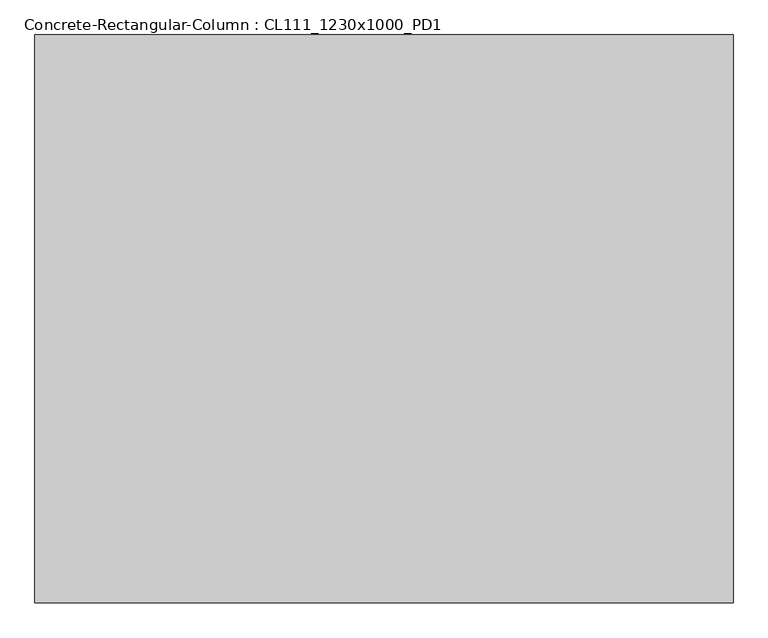
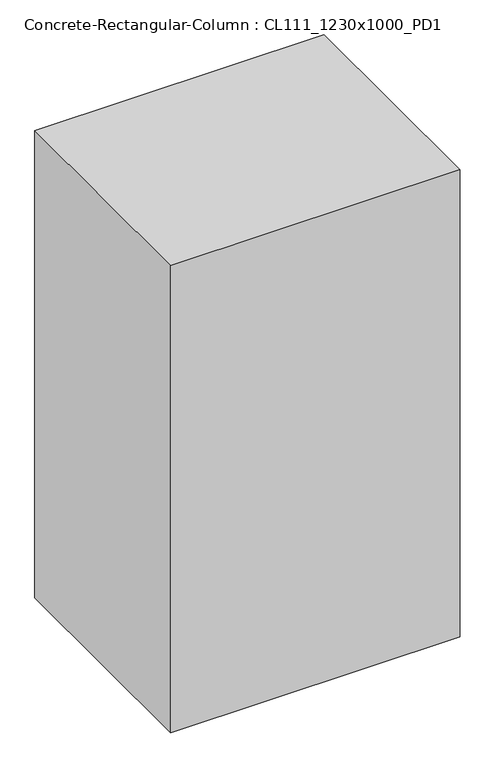
"""IFC4 building model written with IfcOpenShell, lengths in millimetres: column geometry, Concrete-Rectangular-Column : CL111_1230x1000_PD1."""

from ifc_helpers import new_model, si_unit, frame, origin, place, context, project, spatial, polyline, outline, extrude, source, transform, mapped, element, save


def concrete_rectangular_column_cl111_1230x1000_pd1_d73c58a3(model_context):
    return source(origin(), model_context, "Body", "SweptSolid", [
        extrude(outline(polyline([(615.0, 500.0), (615.0, -500.0), (-615.0, -500.0), (-615.0, 500.0), (615.0, 500.0)])), frame((0.0, 0.0, -2100.0), z_axis=(0.0, 0.0, 1.0), x_axis=(1.0, 0.0, 0.0)), (0.0, 0.0, 1.0), 2100.0),
    ])


if __name__ == "__main__":
    model = new_model("IFC4")
    model_context = context("Model", 3, world=origin())
    ifc_project = project(units=[si_unit("LENGTHUNIT", "METRE", prefix="MILLI")], contexts=[model_context])
    site = spatial("IfcSite", under=ifc_project)
    building = spatial("IfcBuilding", under=site)
    placement = place(None, origin())
    concrete_rectangular_column_cl111_1230x1000_pd1_shape = concrete_rectangular_column_cl111_1230x1000_pd1_d73c58a3(model_context)
    element("IfcColumn", 1, ObjectType="Concrete-Rectangular-Column : CL111_1230x1000_PD1", at=placement, inside=building, context=model_context, shape_type="MappedRepresentation", body=[
        mapped(concrete_rectangular_column_cl111_1230x1000_pd1_shape, transform((0.0, 0.0, 0.0), x_axis=(1.0, 0.0, 0.0), y_axis=(0.0, 1.0, 0.0), z_axis=(0.0, 0.0, 1.0))),
    ])
    save(model, "model.ifc")

# Revit data of these elements
# Type "Concrete-Rectangular-Column : CL111_1230x1000_PD1"
#   Description = "UG 철골 기둥용 Pedestal"
#   b = 1230 mm
#   h = 1000 mm
#   Width = 1230 mm
#   Length = 1000 mm
#   hec_material3 [instance default] = none
#   hec_material2 [instance default] = A03AE056-00001_Bitumen/Bituminous/Asphalt Coating
#   hec_material1 [instance default] = A03AC035-00001_Form Work (3 times in use)_Flat
#   Structural Material [instance default] = A03AC032-00007_Structural Concrete_Type1_25MPa-30Mpa
# Element 1 (IfcColumn, "Concrete-Rectangular-Column : CL111_1230x1000_PD1")
#   hec_material2 = none
#   hec_material1 = none
#   Structural Material = 콘크리트 - 현장타설 콘크리트
#   Materials on its faces: "콘크리트 - 현장타설 콘크리트"
# Materials
#   "A03AE056-00001_Bitumen/Bituminous/Asphalt Coating": class "Generic", colour RGB 17 17 17, transparency 0, Description = "Damp-proofing", W00) Work Master Code = "A03AE056-00001", W01) Work Master_Lv1 = "Concrete Work", W02) Work Master_Lv2 = "Concrete Protective Coating (U/G)", W03) Work Master_Spec.1 = "Bitumen/Bituminous/Asphalt Coating", Cost = 0
#   "A03AC035-00001_Form Work (3 times in use)_Flat": class "Wood", colour RGB 149 120 74, transparency 0, Description = "Plywood", W00) Work Master Code = "A03AC035-00001", W01) Work Master_Lv1 = "Concrete Work", W02) Work Master_Lv2 = "Substructure Work", W03) Work Master_Spec.1 = "Form Work (3 times in use)", W04) Work Master_Spec.2 = "Flat Form", W05) Work Master_Spec.3 = "Dressed Lumber, Plywood or Steel Form(Wood Planks are not Allowed) incl. Chamfer", Cost = 0
#   "A03AC032-00007_Structural Concrete_Type1_25MPa-30Mpa": class "Concrete", colour RGB 176 176 176, transparency 0, Keynote = "09910.A1", Description = "Reinf. Conc.", W00) Work Master Code = "A03AC032-00007", W01) Work Master_Lv1 = "Concrete Work", W02) Work Master_Lv2 = "Substructure Work", W03) Work Master_Spec.1 = "Structural Concrete", W04) Work Master_Spec.2 = "Cement Type-1", W05) Work Master_Spec.3 = "25MPa < F'c (Cylinder Strength) ≤ 30MPa", Cost = 0
#   "콘크리트 - 현장타설 콘크리트": class "콘크리트", colour RGB 192 192 192, transparency 0
